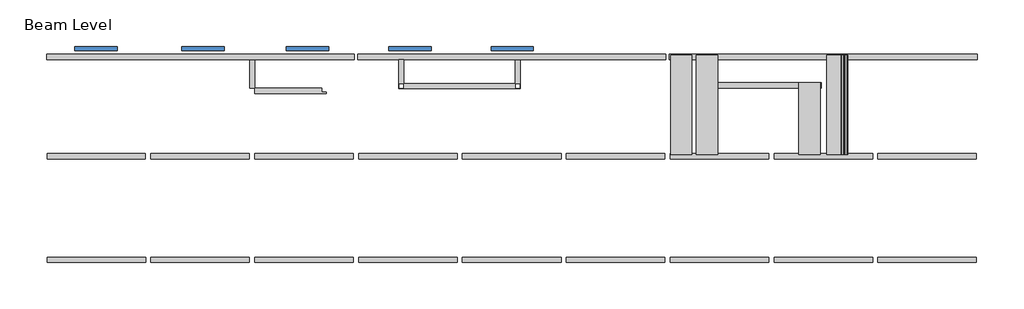
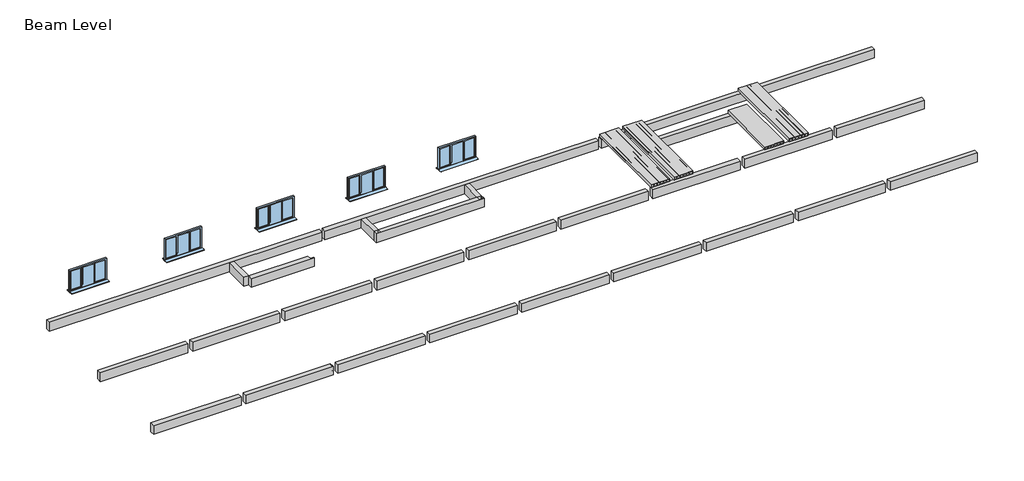
# One storey: 28 beams, 5 windows, 4 proxies.
"""IFC4 building model written with IfcOpenShell, lengths in millimetres."""

import ifcopenshell
import ifcopenshell.guid

model = None  # the IFC model being written
_history = None  # IfcOwnerHistory: only IFC2X3 demands one
_inside = {}  # id of a spatial element -> (the spatial element, [elements in it])
_under = {}  # id of a project, library or spatial element -> (it, [spatial elements below it])
_declared = {}  # id of a project -> (the project, [libraries it declares])
_typed = {}  # id of a type object -> (the type object, [elements of that type])
_made_of = {}  # id of a material, layer set ... -> (it, [elements and type objects made of it])


def new_model(schema):
    """Start an empty IFC model of exactly this schema.

    Asked for "IFC4X3", IfcOpenShell would pick the latest addendum, in which some entities
    have other attributes; the version numbers below select the first issue.
    IFC2X3 requires an IfcOwnerHistory on every rooted entity: one is made here for all.
    """
    global model, _history
    if schema == "IFC4X3":
        model = ifcopenshell.file(schema_version=(4, 3, 0, 0))
    else:
        model = ifcopenshell.file(schema=schema)
    _inside.clear()
    _under.clear()
    _declared.clear()
    _typed.clear()
    _made_of.clear()
    _history = None
    if model.schema == "IFC2X3":
        org = make("IfcOrganization", Name="unknown")
        user = make(
            "IfcPersonAndOrganization",
            ThePerson=make("IfcPerson", FamilyName="unknown"),
            TheOrganization=org,
        )
        app = make(
            "IfcApplication",
            ApplicationDeveloper=org,
            Version="unknown",
            ApplicationFullName="unknown",
            ApplicationIdentifier="unknown",
        )
        _history = make(
            "IfcOwnerHistory",
            OwningUser=user,
            OwningApplication=app,
            ChangeAction="ADDED",
            CreationDate=0,
        )
    return model


def make(cls, **values):
    """One entity of the class cls with the attributes given. An attribute that is None is left unset."""
    return model.create_entity(
        cls, **{name: value for name, value in values.items() if value is not None}
    )


def rooted(cls, **values):
    """An entity with a GlobalId (a new one), such as an element, a storey or a relation."""
    return make(cls, GlobalId=ifcopenshell.guid.new(), OwnerHistory=_history, **values)


def si_unit(unit_type, name, prefix=None):
    """IfcSIUnit, for example si_unit("LENGTHUNIT", "METRE", prefix="MILLI")."""
    return make("IfcSIUnit", UnitType=unit_type, Prefix=prefix, Name=name)


def assignment(units):
    """IfcUnitAssignment: the units of a project."""
    return None if units is None else make("IfcUnitAssignment", Units=units)


def point(xyz):
    """IfcCartesianPoint."""
    return None if xyz is None else make("IfcCartesianPoint", Coordinates=xyz)


def direction(xyz):
    """IfcDirection."""
    return None if xyz is None else make("IfcDirection", DirectionRatios=xyz)


def frame(location, z_axis=None, x_axis=None):
    """IfcAxis2Placement3D, a coordinate frame: its origin and axes. An axis left out is left unset."""
    return make(
        "IfcAxis2Placement3D",
        Location=point(location),
        Axis=direction(z_axis),
        RefDirection=direction(x_axis),
    )


def frame_2d(location, x_axis=None):
    """IfcAxis2Placement2D, a coordinate frame in the plane: its origin and x axis."""
    return make(
        "IfcAxis2Placement2D", Location=point(location), RefDirection=direction(x_axis)
    )


def origin():
    """The frame at (0, 0, 0) with its axes left unset."""
    return frame((0.0, 0.0, 0.0))


def place(relative_to, where):
    """IfcLocalPlacement: puts the frame where relative to a parent placement (None: the world)."""
    return make(
        "IfcLocalPlacement", PlacementRelTo=relative_to, RelativePlacement=where
    )


def context(
    kind, dimensions, precision=None, world=None, true_north=None, identifier=None
):
    """IfcGeometricRepresentationContext, for example the 3D "Model" context."""
    return make(
        "IfcGeometricRepresentationContext",
        ContextIdentifier=identifier,
        ContextType=kind,
        CoordinateSpaceDimension=dimensions,
        Precision=precision,
        WorldCoordinateSystem=world,
        TrueNorth=true_north,
    )


def project(units=None, contexts=None):
    """IfcProject with its units and contexts."""
    return rooted(
        "IfcProject",
        Name="project",
        RepresentationContexts=contexts,
        UnitsInContext=assignment(units),
    )


def spatial(cls, under=None, at=None, **own):
    """A site, building, storey or space (cls), placed at a placement, below another one or the project."""
    s = rooted(cls, ObjectPlacement=at, **own)
    if under is not None:
        _under.setdefault(under.id(), (under, []))[1].append(s)
    return s


def polyline(points):
    """IfcPolyline through the points."""
    return make("IfcPolyline", Points=[point(p) for p in points])


def circle_curve(where, radius):
    """IfcCircle in the frame where."""
    return make("IfcCircle", Position=where, Radius=radius)


def trimmed(basis, trim1, trim2, sense, master):
    """IfcTrimmedCurve: the piece of a basis curve between two trims."""
    return make(
        "IfcTrimmedCurve",
        BasisCurve=basis,
        Trim1=trim1,
        Trim2=trim2,
        SenseAgreement=sense,
        MasterRepresentation=master,
    )


def segment(curve, same_sense, transition):
    """IfcCompositeCurveSegment."""
    return make(
        "IfcCompositeCurveSegment",
        Transition=transition,
        SameSense=same_sense,
        ParentCurve=curve,
    )


def composite_curve(segments, self_intersect=None):
    """IfcCompositeCurve: segments joined end to end."""
    return make("IfcCompositeCurve", Segments=segments, SelfIntersect=self_intersect)


def outline(outer, holes=None, kind="AREA"):
    """IfcArbitraryClosedProfileDef: a profile drawn as a closed curve; with holes, ...WithVoids."""
    if holes is None:
        return make("IfcArbitraryClosedProfileDef", ProfileType=kind, OuterCurve=outer)
    return make(
        "IfcArbitraryProfileDefWithVoids",
        ProfileType=kind,
        OuterCurve=outer,
        InnerCurves=holes,
    )


def extrude(swept, where, along, depth):
    """IfcExtrudedAreaSolid: the profile swept, set in the frame where, extruded along a direction by depth."""
    return make(
        "IfcExtrudedAreaSolid",
        SweptArea=swept,
        Position=where,
        ExtrudedDirection=direction(along),
        Depth=depth,
    )


def faces_of(points, faces, orient=None, outer=None):
    """IfcFace entities. A face is a list of loops; a loop is a list of indices into points, from 0.

    orient and outer hold one flag for each loop. By default every Orientation is true, the
    first loop of a face is its IfcFaceOuterBound and the others are IfcFaceBound.
    """
    made = []
    for i, loops in enumerate(faces):
        bounds = []
        for j, loop in enumerate(loops):
            is_outer = j == 0 if outer is None else outer[i][j]
            bounds.append(
                make(
                    "IfcFaceOuterBound" if is_outer else "IfcFaceBound",
                    Bound=make("IfcPolyLoop", Polygon=[points[k] for k in loop]),
                    Orientation=True if orient is None else orient[i][j],
                )
            )
        made.append(make("IfcFace", Bounds=bounds))
    return made


def faceted_brep(points, faces, orient=None, outer=None, voids=None):
    """IfcFacetedBrep: a solid bounded by flat faces; with voids (closed shells), ...WithVoids."""
    shared = [point(p) for p in points]
    hull = make("IfcClosedShell", CfsFaces=faces_of(shared, faces, orient, outer))
    if voids is None:
        return make("IfcFacetedBrep", Outer=hull)
    return make(
        "IfcFacetedBrepWithVoids",
        Outer=hull,
        Voids=[
            make(cls, CfsFaces=faces_of(shared, fs, o, b)) for cls, fs, o, b in voids
        ],
    )


def shape(context_of_items, identifier, shape_type, items):
    """IfcShapeRepresentation: the items that make up one representation, for example the "Body"."""
    return make(
        "IfcShapeRepresentation",
        ContextOfItems=context_of_items,
        RepresentationIdentifier=identifier,
        RepresentationType=shape_type,
        Items=items,
    )


def source(mapping_origin, context_of_items, identifier, shape_type, items):
    """IfcRepresentationMap: a shape defined once, which mapped items show again and again."""
    return make(
        "IfcRepresentationMap",
        MappingOrigin=mapping_origin,
        MappedRepresentation=shape(context_of_items, identifier, shape_type, items),
    )


def transform(
    local_origin,
    x_axis=None,
    y_axis=None,
    z_axis=None,
    scale=None,
    scale2=None,
    scale3=None,
    uniform=True,
):
    """IfcCartesianTransformationOperator3D, or its non-uniform kind. x_axis, y_axis, z_axis: its Axis1, 2, 3."""
    if uniform:
        return make(
            "IfcCartesianTransformationOperator3D",
            Axis1=direction(x_axis),
            Axis2=direction(y_axis),
            LocalOrigin=point(local_origin),
            Scale=scale,
            Axis3=direction(z_axis),
        )
    return make(
        "IfcCartesianTransformationOperator3DnonUniform",
        Axis1=direction(x_axis),
        Axis2=direction(y_axis),
        LocalOrigin=point(local_origin),
        Scale=scale,
        Axis3=direction(z_axis),
        Scale2=scale2,
        Scale3=scale3,
    )


def mapped(mapping_source, mapping_target):
    """IfcMappedItem: shows the shape of a source again, moved by a transform."""
    return make(
        "IfcMappedItem", MappingSource=mapping_source, MappingTarget=mapping_target
    )


def made_of(thing, what):
    """Note that an element or type object is made of a material, layer set ...; save() writes the relation."""
    if what is not None:
        _made_of.setdefault(what.id(), (what, []))[1].append(thing)
    return thing


def element(
    cls,
    number,
    at=None,
    inside=None,
    cuts=None,
    type_object=None,
    material=None,
    context=None,
    identifier="Body",
    shape_type=None,
    held_by="IfcProductDefinitionShape",
    body=None,
    shapes=None,
    **own,
):
    """One element of the class cls, such as IfcWall. Its Tag is "e" and its number.

    at: its placement. inside: the storey or other place that contains it. cuts: it is an
    opening in that element (IfcRelVoidsElement). A single representation is given by context,
    identifier, shape_type and body (its items); several are given by shapes. held_by: the class
    of the entity that holds the representations. save() writes the other relations.
    """
    e = rooted(cls, Tag="e%d" % number, ObjectPlacement=at, **own)
    if body is not None:
        shapes = [shape(context, identifier, shape_type, body)]
    if shapes is not None:
        e.Representation = make(held_by, Representations=shapes)
    if inside is not None:
        _inside.setdefault(inside.id(), (inside, []))[1].append(e)
    if cuts is not None:
        rooted(
            "IfcRelVoidsElement", RelatingBuildingElement=cuts, RelatedOpeningElement=e
        )
    if type_object is not None:
        _typed.setdefault(type_object.id(), (type_object, []))[1].append(e)
    return made_of(e, material)


def aggregate(whole, parts):
    """IfcRelAggregates: a whole, such as a stair, and the parts it consists of."""
    return rooted("IfcRelAggregates", RelatingObject=whole, RelatedObjects=parts)


def save(model, path):
    """Write the relations noted so far, then the file.

    IfcRelAggregates (storeys below a building ...), IfcRelContainedInSpatialStructure (elements
    in a storey), IfcRelDefinesByType, IfcRelAssociatesMaterial and IfcRelDeclares: one each for
    every whole, place, type object, material and project.
    """
    for whole, parts in _under.values():
        aggregate(whole, parts)
    for where, things in _inside.values():
        rooted(
            "IfcRelContainedInSpatialStructure",
            RelatedElements=things,
            RelatingStructure=where,
        )
    for kind, things in _typed.values():
        rooted("IfcRelDefinesByType", RelatedObjects=things, RelatingType=kind)
    for what, things in _made_of.values():
        rooted("IfcRelAssociatesMaterial", RelatedObjects=things, RelatingMaterial=what)
    for by, libraries in _declared.values():
        rooted("IfcRelDeclares", RelatingContext=by, RelatedDefinitions=libraries)
    model.write(path)


def asb_beams_300asb153_cd404b0f(model_context):
    return source(origin(), model_context, "Body", "SweptSolid", [
        extrude(outline(composite_curve([segment(polyline([(95.0, 174.0), (95.0, 150.0), (40.5, 150.0)]), True, "CONTINUOUS"), segment(trimmed(circle_curve(frame_2d((40.5, 123.0)), 27.0), [point((40.5, 150.0))], [point((13.5, 123.0))], True, "CARTESIAN"), True, "CONTINUOUS"), segment(polyline([(13.5, 123.0), (13.5, -85.0)]), True, "CONTINUOUS"), segment(trimmed(circle_curve(frame_2d((40.5, -85.0)), 27.0), [point((13.5, -85.0))], [point((40.5, -112.0))], True, "CARTESIAN"), True, "CONTINUOUS"), segment(polyline([(40.5, -112.0), (150.0, -112.0), (150.0, -136.0), (-150.0, -136.0), (-150.0, -112.0), (-40.5, -112.0)]), True, "CONTINUOUS"), segment(trimmed(circle_curve(frame_2d((-40.5, -85.0)), 27.0), [point((-40.5, -112.0))], [point((-13.5, -85.0))], True, "CARTESIAN"), True, "CONTINUOUS"), segment(polyline([(-13.5, -85.0), (-13.5, 123.0)]), True, "CONTINUOUS"), segment(trimmed(circle_curve(frame_2d((-40.5, 123.0)), 27.0), [point((-13.5, 123.0))], [point((-40.5, 150.0))], True, "CARTESIAN"), True, "CONTINUOUS"), segment(polyline([(-40.5, 150.0), (-95.0, 150.0), (-95.0, 174.0), (95.0, 174.0)]), True, "CONTINUOUS")], self_intersect=False)), frame((-176.5, 0.0, 0.0), z_axis=(1.0, 0.0, 0.0), x_axis=(0.0, 1.0, 0.0)), (0.0, 0.0, 1.0), 36.0),
    ])


def hollow_core_b1c9e8cf(model_context):
    return source(origin(), model_context, "Body", "SweptSolid", [
        extrude(outline(polyline([(-609.6, 100.0), (609.6, 100.0), (609.6, -100.0), (-609.6, -100.0), (-609.6, 100.0)]), holes=[composite_curve([segment(trimmed(circle_curve(frame_2d((508.0, 0.0)), 60.0), [point((448.0, 0.0))], [point((568.0, 0.0))], True, "CARTESIAN"), True, "CONTINUOUS"), segment(trimmed(circle_curve(frame_2d((508.0, 0.0)), 60.0), [point((568.0, 0.0))], [point((448.0, 0.0))], True, "CARTESIAN"), True, "CONTINUOUS")], self_intersect=False), composite_curve([segment(trimmed(circle_curve(frame_2d((-508.0, 0.0)), 60.0), [point((-568.0, 0.0))], [point((-448.0, 0.0))], True, "CARTESIAN"), True, "CONTINUOUS"), segment(trimmed(circle_curve(frame_2d((-508.0, 0.0)), 60.0), [point((-448.0, 0.0))], [point((-568.0, 0.0))], True, "CARTESIAN"), True, "CONTINUOUS")], self_intersect=False), composite_curve([segment(trimmed(circle_curve(frame_2d((304.8, 0.0)), 60.0), [point((244.8, 0.0))], [point((364.8, 0.0))], True, "CARTESIAN"), True, "CONTINUOUS"), segment(trimmed(circle_curve(frame_2d((304.8, 0.0)), 60.0), [point((364.8, 0.0))], [point((244.8, 0.0))], True, "CARTESIAN"), True, "CONTINUOUS")], self_intersect=False), composite_curve([segment(trimmed(circle_curve(frame_2d((101.6, 0.0)), 60.0), [point((41.6, 0.0))], [point((161.6, 0.0))], True, "CARTESIAN"), True, "CONTINUOUS"), segment(trimmed(circle_curve(frame_2d((101.6, 0.0)), 60.0), [point((161.6, 0.0))], [point((41.6, 0.0))], True, "CARTESIAN"), True, "CONTINUOUS")], self_intersect=False), composite_curve([segment(trimmed(circle_curve(frame_2d((-101.6, 0.0)), 60.0), [point((-161.6, 0.0))], [point((-41.6, 0.0))], True, "CARTESIAN"), True, "CONTINUOUS"), segment(trimmed(circle_curve(frame_2d((-101.6, 0.0)), 60.0), [point((-41.6, 0.0))], [point((-161.6, 0.0))], True, "CARTESIAN"), True, "CONTINUOUS")], self_intersect=False), composite_curve([segment(trimmed(circle_curve(frame_2d((-304.8, 0.0)), 60.0), [point((-364.8, 0.0))], [point((-244.8, 0.0))], True, "CARTESIAN"), True, "CONTINUOUS"), segment(trimmed(circle_curve(frame_2d((-304.8, 0.0)), 60.0), [point((-244.8, 0.0))], [point((-364.8, 0.0))], True, "CARTESIAN"), True, "CONTINUOUS")], self_intersect=False)]), frame((0.0, 0.0, 0.0), z_axis=(1.0, 0.0, 0.0), x_axis=(0.0, 1.0, 0.0)), (0.0, 0.0, 1.0), 5760.0),
    ])


def hollow_core_a6975cb3(model_context):
    return source(origin(), model_context, "Body", "SweptSolid", [
        extrude(outline(polyline([(-609.6, 100.0), (609.6, 100.0), (609.6, -100.0), (-609.6, -100.0), (-609.6, 100.0)]), holes=[composite_curve([segment(trimmed(circle_curve(frame_2d((508.0, 0.0)), 60.0), [point((448.0, 0.0))], [point((568.0, 0.0))], True, "CARTESIAN"), True, "CONTINUOUS"), segment(trimmed(circle_curve(frame_2d((508.0, 0.0)), 60.0), [point((568.0, 0.0))], [point((448.0, 0.0))], True, "CARTESIAN"), True, "CONTINUOUS")], self_intersect=False), composite_curve([segment(trimmed(circle_curve(frame_2d((-508.0, 0.0)), 60.0), [point((-568.0, 0.0))], [point((-448.0, 0.0))], True, "CARTESIAN"), True, "CONTINUOUS"), segment(trimmed(circle_curve(frame_2d((-508.0, 0.0)), 60.0), [point((-448.0, 0.0))], [point((-568.0, 0.0))], True, "CARTESIAN"), True, "CONTINUOUS")], self_intersect=False), composite_curve([segment(trimmed(circle_curve(frame_2d((304.8, 0.0)), 60.0), [point((244.8, 0.0))], [point((364.8, 0.0))], True, "CARTESIAN"), True, "CONTINUOUS"), segment(trimmed(circle_curve(frame_2d((304.8, 0.0)), 60.0), [point((364.8, 0.0))], [point((244.8, 0.0))], True, "CARTESIAN"), True, "CONTINUOUS")], self_intersect=False), composite_curve([segment(trimmed(circle_curve(frame_2d((101.6, 0.0)), 60.0), [point((41.6, 0.0))], [point((161.6, 0.0))], True, "CARTESIAN"), True, "CONTINUOUS"), segment(trimmed(circle_curve(frame_2d((101.6, 0.0)), 60.0), [point((161.6, 0.0))], [point((41.6, 0.0))], True, "CARTESIAN"), True, "CONTINUOUS")], self_intersect=False), composite_curve([segment(trimmed(circle_curve(frame_2d((-101.6, 0.0)), 60.0), [point((-161.6, 0.0))], [point((-41.6, 0.0))], True, "CARTESIAN"), True, "CONTINUOUS"), segment(trimmed(circle_curve(frame_2d((-101.6, 0.0)), 60.0), [point((-41.6, 0.0))], [point((-161.6, 0.0))], True, "CARTESIAN"), True, "CONTINUOUS")], self_intersect=False), composite_curve([segment(trimmed(circle_curve(frame_2d((-304.8, 0.0)), 60.0), [point((-364.8, 0.0))], [point((-244.8, 0.0))], True, "CARTESIAN"), True, "CONTINUOUS"), segment(trimmed(circle_curve(frame_2d((-304.8, 0.0)), 60.0), [point((-244.8, 0.0))], [point((-364.8, 0.0))], True, "CARTESIAN"), True, "CONTINUOUS")], self_intersect=False)]), frame((0.0, 0.0, 0.0), z_axis=(1.0, 0.0, 0.0), x_axis=(0.0, 1.0, 0.0)), (0.0, 0.0, 1.0), 4157.5),
    ])


def windows_commercial_ff_rear_windows_2400long_x_1500high_d88e899e(model_context):
    return source(origin(), model_context, "Body", "SolidModel", [
        extrude(outline(polyline([(-1860.0, -231.5434322), (-1860.0, -138.5434322), (-1860.0, 8.4565678), (590.0, 8.4565678), (590.0, -138.5434322), (590.0, -231.5434322), (-1860.0, -231.5434322)])), frame((0.0, 0.0, 636.5715519), z_axis=(0.0, 0.0, 1.0), x_axis=(1.0, 0.0, 0.0)), (0.0, 0.0, 1.0), 26.4284481),
        extrude(outline(polyline([(495.0, 87.4565678), (-190.0, 87.4565678), (-190.0, 111.4565678), (495.0, 111.4565678), (495.0, 87.4565678)])), frame((0.0, 0.0, 693.0), z_axis=(0.0, 0.0, 1.0), x_axis=(1.0, 0.0, 0.0)), (0.0, 0.0, 1.0), 1337.0),
        extrude(outline(polyline([(-1020.0, 47.4565678), (-250.0, 47.4565678), (-250.0, 23.4565678), (-1020.0, 23.4565678), (-1020.0, 47.4565678)])), frame((0.0, 0.0, 663.0), z_axis=(0.0, 0.0, 1.0), x_axis=(1.0, 0.0, 0.0)), (0.0, 0.0, 1.0), 1397.0),
        extrude(outline(polyline([(-1080.0, 87.4565678), (-1765.0, 87.4565678), (-1765.0, 111.4565678), (-1080.0, 111.4565678), (-1080.0, 87.4565678)])), frame((0.0, 0.0, 693.0), z_axis=(0.0, 0.0, 1.0), x_axis=(1.0, 0.0, 0.0)), (0.0, 0.0, 1.0), 1337.0),
        faceted_brep([(-1835.0, 5.4565678, 663.0), (-1775.0, 5.4565678, 663.0), (-1775.0, 5.4565678, 2040.0), (-1068.0, 5.4565678, 2040.0), (-1068.0, 5.4565678, 863.0), (-1010.0, 5.4565678, 863.0), (-1010.0, 5.4565678, 2040.0), (-260.0, 5.4565678, 2040.0), (-260.0, 5.4565678, 663.0), (-202.0, 5.4565678, 663.0), (-202.0, 5.4565678, 2040.0), (505.0, 5.4565678, 2040.0), (505.0, 5.4565678, 663.0), (565.0, 5.4565678, 663.0), (565.0, 5.4565678, 2100.0), (-1835.0, 5.4565678, 2100.0), (-1835.0, 123.4565678, 2100.0), (-1835.0, 123.4565678, 663.0), (-1835.0, 73.4565678, 663.0), (-1835.0, 8.4565678, 663.0), (-1795.0, 123.4565678, 663.0), (565.0, 123.4565678, 2100.0), (565.0, 123.4565678, 663.0), (525.0, 123.4565678, 663.0), (525.0, 123.4565678, 2060.0), (-220.0, 123.4565678, 2060.0), (-220.0, 123.4565678, 663.0), (-260.0, 123.4565678, 663.0), (-260.0, 123.4565678, 2060.0), (-1010.0, 123.4565678, 2060.0), (-1010.0, 123.4565678, 863.0), (-1050.0, 123.4565678, 863.0), (-1050.0, 123.4565678, 2060.0), (-1795.0, 123.4565678, 2060.0), (-1795.0, 23.4565678, 2060.0), (-1795.0, 23.4565678, 663.0), (-1795.0, 73.4565678, 663.0), (-1050.0, 23.4565678, 2060.0), (-1050.0, 23.4565678, 863.0), (-1068.0, 23.4565678, 863.0), (-1068.0, 23.4565678, 2040.0), (-1775.0, 23.4565678, 2040.0), (-1775.0, 23.4565678, 663.0), (525.0, 23.4565678, 2060.0), (525.0, 23.4565678, 663.0), (505.0, 23.4565678, 663.0), (505.0, 23.4565678, 2040.0), (-202.0, 23.4565678, 2040.0), (-202.0, 23.4565678, 663.0), (-220.0, 23.4565678, 663.0), (-220.0, 23.4565678, 2060.0), (-1010.0, 23.4565678, 863.0), (-1020.0, 23.4565678, 863.0), (-1020.0, 23.4565678, 2060.0), (-250.0, 23.4565678, 2060.0), (-250.0, 23.4565678, 663.0), (-260.0, 23.4565678, 663.0), (-260.0, 23.4565678, 2040.0), (-1010.0, 23.4565678, 2040.0), (-1775.0, 8.4565678, 663.0), (-1010.0, 47.4565678, 2060.0), (-260.0, 47.4565678, 2060.0), (-250.0, 47.4565678, 2060.0), (-1020.0, 47.4565678, 2060.0), (565.0, 8.4565678, 663.0), (565.0, 73.4565678, 663.0), (525.0, 73.4565678, 663.0), (505.0, 8.4565678, 663.0), (-1010.0, 47.4565678, 863.0), (-1020.0, 47.4565678, 863.0), (-250.0, 47.4565678, 663.0), (-260.0, 47.4565678, 663.0), (-260.0, 73.4565678, 663.0), (-220.0, 73.4565678, 663.0), (-202.0, 8.4565678, 663.0), (-260.0, 8.4565678, 663.0), (590.0, 248.4565678, 600.0), (590.0, 8.4565678, 600.0), (-1860.0, 8.4565678, 600.0), (-1860.0, 248.4565678, 600.0), (590.0, 248.4565678, 637.0666405), (-1860.0, 248.4565678, 637.0666405), (590.0, 73.4565678, 649.0962075), (-1860.0, 73.4565678, 649.0962075), (590.0, 8.4565678, 663.0), (590.0, 73.4565678, 663.0), (-1860.0, 73.4565678, 663.0), (-1860.0, 8.4565678, 663.0)], [[[0, 1, 2, 3, 4, 5, 6, 7, 8, 9, 10, 11, 12, 13, 14, 15]], [[0, 15, 16, 17, 18, 19]], [[20, 17, 16, 21, 22, 23, 24, 25, 26, 27, 28, 29, 30, 31, 32, 33]], [[20, 33, 34, 35, 36]], [[35, 34, 37, 38, 39, 40, 41, 42]], [[43, 44, 45, 46, 47, 48, 49, 50]], [[51, 52, 53, 54, 55, 56, 57, 58]], [[2, 1, 59, 42, 41]], [[15, 14, 21, 16]], [[34, 33, 32, 37]], [[24, 43, 50, 25]], [[60, 29, 28, 61, 62, 54, 53, 63]], [[2, 41, 40, 3]], [[46, 11, 10, 47]], [[6, 58, 57, 7]], [[14, 13, 64, 65, 22, 21]], [[24, 23, 66, 44, 43]], [[12, 11, 46, 45, 67]], [[5, 51, 58, 6]], [[39, 4, 3, 40]], [[31, 38, 37, 32]], [[68, 30, 29, 60]], [[69, 68, 60, 63]], [[52, 69, 63, 53]], [[62, 70, 55, 54]], [[70, 62, 61, 71]], [[71, 61, 28, 27, 72]], [[26, 25, 50, 49, 73]], [[10, 9, 74, 48, 47]], [[8, 7, 57, 56, 75]], [[76, 77, 78, 79]], [[80, 76, 79, 81]], [[82, 80, 81, 83]], [[84, 85, 65, 64]], [[86, 87, 19, 18]], [[72, 36, 35, 42, 59, 75, 56, 55, 70, 71]], [[66, 73, 49, 48, 74, 67, 45, 44]], [[17, 20, 36, 18]], [[1, 0, 19, 59]], [[23, 22, 65, 66]], [[13, 12, 67, 64]], [[51, 5, 4, 39, 38, 31, 30, 68, 69, 52]], [[27, 26, 73, 72]], [[9, 8, 75, 74]], [[84, 77, 76, 80, 82, 85]], [[87, 86, 83, 81, 79, 78]], [[85, 82, 83, 86, 18, 36, 72, 73, 66, 65]], [[77, 84, 64, 67, 74, 75, 59, 19, 87, 78]]]),
        faceted_brep([(-1050.0, 23.4565678, 2060.0), (-1050.0, 93.4565678, 2060.0), (-1795.0, 93.4565678, 2060.0), (-1795.0, 23.4565678, 2060.0), (-1090.0, 37.9494677, 2020.0), (-1079.8519623, 23.4565678, 2030.1480377), (-1765.1480377, 23.4565678, 2030.1480377), (-1755.0, 37.9494677, 2020.0), (-1090.0, 87.4565678, 2020.0), (-1755.0, 87.4565678, 2020.0), (-1080.0, 111.4565678, 2030.0), (-1080.0, 87.4565678, 2030.0), (-1765.0, 87.4565678, 2030.0), (-1765.0, 111.4565678, 2030.0), (-1090.0, 129.2300705, 2020.0), (-1090.0, 111.4565678, 2020.0), (-1755.0, 111.4565678, 2020.0), (-1755.0, 129.2300705, 2020.0), (-1071.1854344, 135.0035732, 2038.8145656), (-1773.8145656, 135.0035732, 2038.8145656), (-1795.0, 93.4565678, 663.0), (-1795.0, 23.4565678, 663.0), (-1765.1480377, 23.4565678, 692.8519623), (-1755.0, 37.9494677, 703.0), (-1755.0, 87.4565678, 703.0), (-1765.0, 87.4565678, 693.0), (-1765.0, 111.4565678, 693.0), (-1755.0, 111.4565678, 703.0), (-1755.0, 129.2300705, 703.0), (-1773.8145656, 135.0035732, 684.1854344), (-1050.0, 93.4565678, 663.0), (-1050.0, 23.4565678, 663.0), (-1079.8519623, 23.4565678, 692.8519623), (-1090.0, 37.9494677, 703.0), (-1090.0, 87.4565678, 703.0), (-1080.0, 87.4565678, 693.0), (-1080.0, 111.4565678, 693.0), (-1090.0, 111.4565678, 703.0), (-1090.0, 129.2300705, 703.0), (-1071.1854344, 135.0035732, 684.1854344), (-1040.0, 135.0035732, 653.0), (-1805.0, 135.0035732, 653.0), (-1805.0, 135.0035732, 2070.0), (-1040.0, 135.0035732, 2070.0), (-1040.0, 93.4565678, 2070.0), (-1805.0, 93.4565678, 2070.0), (-1805.0, 93.4565678, 653.0), (-1040.0, 93.4565678, 653.0)], [[[0, 1, 2, 3]], [[4, 5, 6, 7]], [[8, 4, 7, 9]], [[10, 11, 12, 13]], [[14, 15, 16, 17]], [[18, 14, 17, 19]], [[3, 2, 20, 21]], [[7, 6, 22, 23]], [[9, 7, 23, 24]], [[13, 12, 25, 26]], [[17, 16, 27, 28]], [[19, 17, 28, 29]], [[21, 20, 30, 31]], [[0, 3, 21, 31], [32, 22, 6, 5]], [[23, 22, 32, 33]], [[24, 23, 33, 34]], [[35, 25, 12, 11], [8, 9, 24, 34]], [[26, 25, 35, 36]], [[10, 13, 26, 36], [37, 27, 16, 15]], [[28, 27, 37, 38]], [[29, 28, 38, 39]], [[40, 41, 42, 43], [18, 19, 29, 39]], [[30, 1, 0, 31]], [[33, 32, 5, 4]], [[34, 33, 4, 8]], [[36, 35, 11, 10]], [[38, 37, 15, 14]], [[39, 38, 14, 18]], [[44, 43, 42, 45]], [[45, 42, 41, 46]], [[46, 41, 40, 47]], [[47, 40, 43, 44]], [[45, 46, 47, 44], [1, 30, 20, 2]]]),
        faceted_brep([(-230.0, 87.4565678, 2070.0), (-230.0, 129.2300705, 2070.0), (-230.0, 129.2300705, 653.0), (-230.0, 87.4565678, 653.0), (-220.0, 23.4565678, 2060.0), (-220.0, 87.4565678, 2060.0), (-220.0, 87.4565678, 663.0), (-220.0, 23.4565678, 663.0), (-180.0, 37.9494677, 2020.0), (-190.1480377, 23.4565678, 2030.1480377), (-190.1480377, 23.4565678, 692.8519623), (-180.0, 37.9494677, 703.0), (-180.0, 87.4565678, 2020.0), (-180.0, 87.4565678, 703.0), (-190.0, 111.4565678, 2030.0), (-190.0, 87.4565678, 2030.0), (-190.0, 87.4565678, 693.0), (-190.0, 111.4565678, 693.0), (-180.0, 129.2300705, 2020.0), (-180.0, 111.4565678, 2020.0), (-180.0, 111.4565678, 703.0), (-180.0, 129.2300705, 703.0), (-197.4457548, 135.0035732, 2037.4457548), (-197.4457548, 135.0035732, 685.5542452), (-219.2153903, 135.0035732, 2059.2153903), (-219.2153903, 135.0035732, 663.7846097), (535.0, 129.2300705, 653.0), (535.0, 87.4565678, 653.0), (525.0, 87.4565678, 663.0), (525.0, 23.4565678, 663.0), (495.1480377, 23.4565678, 692.8519623), (485.0, 37.9494677, 703.0), (485.0, 87.4565678, 703.0), (495.0, 87.4565678, 693.0), (495.0, 111.4565678, 693.0), (485.0, 111.4565678, 703.0), (485.0, 129.2300705, 703.0), (502.4457548, 135.0035732, 685.5542452), (524.2153903, 135.0035732, 663.7846097), (535.0, 129.2300705, 2070.0), (535.0, 87.4565678, 2070.0), (525.0, 87.4565678, 2060.0), (525.0, 23.4565678, 2060.0), (495.1480377, 23.4565678, 2030.1480377), (485.0, 37.9494677, 2020.0), (485.0, 87.4565678, 2020.0), (495.0, 87.4565678, 2030.0), (495.0, 111.4565678, 2030.0), (485.0, 111.4565678, 2020.0), (485.0, 129.2300705, 2020.0), (502.4457548, 135.0035732, 2037.4457548), (524.2153903, 135.0035732, 2059.2153903)], [[[0, 1, 2, 3]], [[4, 5, 6, 7]], [[8, 9, 10, 11]], [[12, 8, 11, 13]], [[14, 15, 16, 17]], [[18, 19, 20, 21]], [[22, 18, 21, 23]], [[1, 24, 25, 2]], [[3, 2, 26, 27]], [[7, 6, 28, 29]], [[11, 10, 30, 31]], [[13, 11, 31, 32]], [[17, 16, 33, 34]], [[21, 20, 35, 36]], [[23, 21, 36, 37]], [[2, 25, 38, 26]], [[27, 26, 39, 40]], [[29, 28, 41, 42]], [[31, 30, 43, 44]], [[32, 31, 44, 45]], [[34, 33, 46, 47]], [[36, 35, 48, 49]], [[37, 36, 49, 50]], [[26, 38, 51, 39]], [[40, 39, 1, 0]], [[42, 41, 5, 4]], [[7, 29, 42, 4], [9, 43, 30, 10]], [[44, 43, 9, 8]], [[45, 44, 8, 12]], [[15, 46, 33, 16], [13, 32, 45, 12]], [[47, 46, 15, 14]], [[17, 34, 47, 14], [19, 48, 35, 20]], [[49, 48, 19, 18]], [[50, 49, 18, 22]], [[24, 51, 38, 25], [23, 37, 50, 22]], [[39, 51, 24, 1]], [[3, 27, 40, 0], [5, 41, 28, 6]]]),
    ])


model = new_model("IFC4")

# Units and contexts
model_context = context("Model", 3, world=origin())
ifc_project = project(units=[si_unit("LENGTHUNIT", "METRE", prefix="MILLI")], contexts=[model_context])

# Site, building, storey
site = spatial("IfcSite", under=ifc_project)
building = spatial("IfcBuilding", under=site)
storey = spatial("IfcBuildingStorey", under=building, Name="Beam Level", Elevation=3700.0)

# Beams
placement = place(None, origin())
asb_beams_300asb153_shape = asb_beams_300asb153_cd404b0f(model_context)
element("IfcBeam", 1, ObjectType="ASB-Beams : 300ASB153", at=placement, inside=storey, context=model_context, shape_type="MappedRepresentation", body=[
    mapped(asb_beams_300asb153_shape, transform((4837.4196543, -5058.7619082, 3526.0), x_axis=(1.0, 0.0, 0.0), y_axis=(0.0, 1.0, 0.0), z_axis=(0.0, 0.0, 1.0))),
])
element("IfcBeam", 2, ObjectType="Concrete - Rectangular Beam : 300 x 600mm", at=placement, inside=storey, context=model_context, shape_type="SweptSolid", body=[
    extrude(outline(polyline([(-1300.8053457, 1091.2380918), (-1300.8053457, 791.2380918), (-6985.5053457, 791.2380918), (-6985.5053457, 1091.2380918), (-1300.8053457, 1091.2380918)])), frame((0.0, 0.0, 3100.0), z_axis=(0.0, 0.0, 1.0), x_axis=(1.0, 0.0, 0.0)), (0.0, 0.0, 1.0), 600.0),
])
element("IfcBeam", 3, ObjectType="Concrete - Rectangular Beam : 300 x 600mm", at=placement, inside=storey, context=model_context, shape_type="SweptSolid", body=[
    extrude(outline(polyline([(-985.6053457, 791.2380918), (-985.6053457, 1091.2380918), (4710.4446543, 1091.2380918), (4710.4446543, 791.2380918), (-985.6053457, 791.2380918)])), frame((0.0, 0.0, 3100.0), z_axis=(0.0, 0.0, 1.0), x_axis=(1.0, 0.0, 0.0)), (0.0, 0.0, 1.0), 600.0),
])
element("IfcBeam", 4, ObjectType="Concrete - Rectangular Beam : 300 x 600mm", at=placement, inside=storey, context=model_context, shape_type="SweptSolid", body=[
    extrude(outline(polyline([(10706.1946543, 1091.2380918), (10706.1946543, 791.2380918), (5010.4446543, 791.2380918), (5010.4446543, 1091.2380918), (10706.1946543, 1091.2380918)])), frame((0.0, 0.0, 3100.0), z_axis=(0.0, 0.0, 1.0), x_axis=(1.0, 0.0, 0.0)), (0.0, 0.0, 1.0), 600.0),
])
element("IfcBeam", 5, ObjectType="Concrete - Rectangular Beam : 300 x 600mm", at=placement, inside=storey, context=model_context, shape_type="SweptSolid", body=[
    extrude(outline(polyline([(-6985.3053457, -5208.7619082), (-6985.3053457, -4908.7619082), (-1289.5553457, -4908.7619082), (-1289.5553457, -5208.7619082), (-6985.3053457, -5208.7619082)])), frame((0.0, 0.0, 3100.0), z_axis=(0.0, 0.0, 1.0), x_axis=(1.0, 0.0, 0.0)), (0.0, 0.0, 1.0), 600.0),
])
element("IfcBeam", 6, ObjectType="Concrete - Rectangular Beam : 300 x 600mm", at=placement, inside=storey, context=model_context, shape_type="SweptSolid", body=[
    extrude(outline(polyline([(-985.6053457, -5208.7619082), (-985.6053457, -4908.7619082), (4710.4446543, -4908.7619082), (4710.4446543, -5208.7619082), (-985.6053457, -5208.7619082)])), frame((0.0, 0.0, 3100.0), z_axis=(0.0, 0.0, 1.0), x_axis=(1.0, 0.0, 0.0)), (0.0, 0.0, 1.0), 600.0),
])
element("IfcBeam", 7, ObjectType="Concrete - Rectangular Beam : 300 x 600mm", at=placement, inside=storey, context=model_context, shape_type="SweptSolid", body=[
    extrude(outline(polyline([(10706.1946543, -4908.7619082), (10706.1946543, -5208.7619082), (5010.4446543, -5208.7619082), (5010.4446543, -4908.7619082), (10706.1946543, -4908.7619082)])), frame((0.0, 0.0, 3100.0), z_axis=(0.0, 0.0, 1.0), x_axis=(1.0, 0.0, 0.0)), (0.0, 0.0, 1.0), 600.0),
])
element("IfcBeam", 8, ObjectType="Concrete - Rectangular Beam : 300 x 600mm", at=placement, inside=storey, context=model_context, shape_type="SweptSolid", body=[
    extrude(outline(polyline([(16699.1946543, 1091.2380918), (16699.1946543, 791.2380918), (11014.4946543, 791.2380918), (11014.4946543, 1091.2380918), (16699.1946543, 1091.2380918)])), frame((0.0, 0.0, 3100.0), z_axis=(0.0, 0.0, 1.0), x_axis=(1.0, 0.0, 0.0)), (0.0, 0.0, 1.0), 600.0),
])
element("IfcBeam", 9, ObjectType="Concrete - Rectangular Beam : 300 x 600mm", at=placement, inside=storey, context=model_context, shape_type="SweptSolid", body=[
    extrude(outline(polyline([(17014.3946543, 791.2380918), (17014.3946543, 1091.2380918), (22710.4446543, 1091.2380918), (22710.4446543, 791.2380918), (17014.3946543, 791.2380918)])), frame((0.0, 0.0, 3100.0), z_axis=(0.0, 0.0, 1.0), x_axis=(1.0, 0.0, 0.0)), (0.0, 0.0, 1.0), 600.0),
])
element("IfcBeam", 10, ObjectType="Concrete - Rectangular Beam : 300 x 600mm", at=placement, inside=storey, context=model_context, shape_type="SweptSolid", body=[
    extrude(outline(polyline([(28706.1946543, 1091.2380918), (28706.1946543, 791.2380918), (23010.4446543, 791.2380918), (23010.4446543, 1091.2380918), (28706.1946543, 1091.2380918)])), frame((0.0, 0.0, 3100.0), z_axis=(0.0, 0.0, 1.0), x_axis=(1.0, 0.0, 0.0)), (0.0, 0.0, 1.0), 600.0),
])
element("IfcBeam", 11, ObjectType="Concrete - Rectangular Beam : 300 x 600mm", at=placement, inside=storey, context=model_context, shape_type="SweptSolid", body=[
    extrude(outline(polyline([(11014.6946543, -5208.7619082), (11014.6946543, -4908.7619082), (16710.4446543, -4908.7619082), (16710.4446543, -5208.7619082), (11014.6946543, -5208.7619082)])), frame((0.0, 0.0, 3100.0), z_axis=(0.0, 0.0, 1.0), x_axis=(1.0, 0.0, 0.0)), (0.0, 0.0, 1.0), 600.0),
])
element("IfcBeam", 12, ObjectType="Concrete - Rectangular Beam : 300 x 600mm", at=placement, inside=storey, context=model_context, shape_type="SweptSolid", body=[
    extrude(outline(polyline([(17014.3946543, -5208.7619082), (17014.3946543, -4908.7619082), (22710.4446543, -4908.7619082), (22710.4446543, -5208.7619082), (17014.3946543, -5208.7619082)])), frame((0.0, 0.0, 3100.0), z_axis=(0.0, 0.0, 1.0), x_axis=(1.0, 0.0, 0.0)), (0.0, 0.0, 1.0), 600.0),
])
element("IfcBeam", 13, ObjectType="Concrete - Rectangular Beam : 300 x 600mm", at=placement, inside=storey, context=model_context, shape_type="SweptSolid", body=[
    extrude(outline(polyline([(28706.1946543, -4908.7619082), (28706.1946543, -5208.7619082), (23010.4446543, -5208.7619082), (23010.4446543, -4908.7619082), (28706.1946543, -4908.7619082)])), frame((0.0, 0.0, 3100.0), z_axis=(0.0, 0.0, 1.0), x_axis=(1.0, 0.0, 0.0)), (0.0, 0.0, 1.0), 600.0),
])
element("IfcBeam", 14, ObjectType="Concrete - Rectangular Beam : 300 x 600mm", at=placement, inside=storey, context=model_context, shape_type="SweptSolid", body=[
    extrude(outline(polyline([(34699.1946543, 1091.2380918), (34699.1946543, 791.2380918), (29014.4946543, 791.2380918), (29014.4946543, 1091.2380918), (34699.1946543, 1091.2380918)])), frame((0.0, 0.0, 3100.0), z_axis=(0.0, 0.0, 1.0), x_axis=(1.0, 0.0, 0.0)), (0.0, 0.0, 1.0), 600.0),
])
element("IfcBeam", 15, ObjectType="Concrete - Rectangular Beam : 300 x 600mm", at=placement, inside=storey, context=model_context, shape_type="SweptSolid", body=[
    extrude(outline(polyline([(35014.3946543, 791.2380918), (35014.3946543, 1091.2380918), (40710.4446543, 1091.2380918), (40710.4446543, 791.2380918), (35014.3946543, 791.2380918)])), frame((0.0, 0.0, 3100.0), z_axis=(0.0, 0.0, 1.0), x_axis=(1.0, 0.0, 0.0)), (0.0, 0.0, 1.0), 600.0),
])
element("IfcBeam", 16, ObjectType="Concrete - Rectangular Beam : 300 x 600mm", at=placement, inside=storey, context=model_context, shape_type="SweptSolid", body=[
    extrude(outline(polyline([(46706.1946543, 1091.2380918), (46706.1946543, 791.2380918), (41010.4446543, 791.2380918), (41010.4446543, 1091.2380918), (46706.1946543, 1091.2380918)])), frame((0.0, 0.0, 3100.0), z_axis=(0.0, 0.0, 1.0), x_axis=(1.0, 0.0, 0.0)), (0.0, 0.0, 1.0), 600.0),
])
element("IfcBeam", 17, ObjectType="Concrete - Rectangular Beam : 300 x 600mm", at=placement, inside=storey, context=model_context, shape_type="SweptSolid", body=[
    extrude(outline(polyline([(29014.6946543, -5208.7619082), (29014.6946543, -4908.7619082), (34710.4446543, -4908.7619082), (34710.4446543, -5208.7619082), (29014.6946543, -5208.7619082)])), frame((0.0, 0.0, 3100.0), z_axis=(0.0, 0.0, 1.0), x_axis=(1.0, 0.0, 0.0)), (0.0, 0.0, 1.0), 600.0),
])
element("IfcBeam", 18, ObjectType="Concrete - Rectangular Beam : 300 x 600mm", at=placement, inside=storey, context=model_context, shape_type="SweptSolid", body=[
    extrude(outline(polyline([(35014.3946543, -5208.7619082), (35014.3946543, -4908.7619082), (40710.4446543, -4908.7619082), (40710.4446543, -5208.7619082), (35014.3946543, -5208.7619082)])), frame((0.0, 0.0, 3100.0), z_axis=(0.0, 0.0, 1.0), x_axis=(1.0, 0.0, 0.0)), (0.0, 0.0, 1.0), 600.0),
])
element("IfcBeam", 19, ObjectType="Concrete - Rectangular Beam : 300 x 600mm", at=placement, inside=storey, context=model_context, shape_type="SweptSolid", body=[
    extrude(outline(polyline([(46705.4946543, -4908.7619082), (46705.4946543, -5208.7619082), (41010.4446543, -5208.7619082), (41010.4446543, -4908.7619082), (46705.4946543, -4908.7619082)])), frame((0.0, 0.0, 3100.0), z_axis=(0.0, 0.0, 1.0), x_axis=(1.0, 0.0, 0.0)), (0.0, 0.0, 1.0), 600.0),
])
element("IfcBeam", 20, ObjectType="Concrete - Rectangular Beam : 300 x 600mm", at=placement, inside=storey, context=model_context, shape_type="Brep", body=[
    faceted_brep([(10765.2696543, 6833.7380918, 3700.0), (10765.2696543, 6533.7380918, 3700.0), (10765.2696543, 6533.7380918, 3100.0), (10765.2696543, 6833.7380918, 3100.0), (-7013.1303457, 6833.7380918, 3700.0), (-7013.1303457, 6833.7380918, 3100.0), (-7013.1303457, 6533.7380918, 3100.0), (-7013.1303457, 6533.7380918, 3700.0), (4722.9446543, 6533.7380918, 3700.0), (5022.9446543, 6533.7380918, 3700.0), (4722.9446543, 6533.7380918, 3100.0), (5022.9446543, 6533.7380918, 3100.0)], [[[0, 1, 2, 3]], [[4, 5, 6, 7]], [[1, 0, 4, 7, 8, 9]], [[2, 1, 9, 8, 7, 6, 10, 11]], [[3, 2, 11, 10, 6, 5]], [[0, 3, 5, 4]]]),
])
element("IfcBeam", 21, ObjectType="Concrete - Rectangular Beam : 300 x 600mm", at=placement, inside=storey, context=model_context, shape_type="Brep", body=[
    faceted_brep([(28765.6446543, 6833.7380918, 3700.0), (28765.6446543, 6533.7380918, 3700.0), (28765.6446543, 6533.7380918, 3100.0), (28765.6446543, 6833.7380918, 3100.0), (10960.2446543, 6833.7380918, 3700.0), (10960.2446543, 6833.7380918, 3100.0), (10960.2446543, 6533.7380918, 3100.0), (10960.2446543, 6533.7380918, 3700.0), (13322.5475614, 6533.7380918, 3700.0), (13622.5475614, 6533.7380918, 3700.0), (20056.9831159, 6533.7380918, 3700.0), (20356.9831159, 6533.7380918, 3700.0), (13322.5475614, 6533.7380918, 3100.0), (13622.5475614, 6533.7380918, 3100.0), (20056.9831159, 6533.7380918, 3100.0), (20356.9831159, 6533.7380918, 3100.0)], [[[0, 1, 2, 3]], [[4, 5, 6, 7]], [[1, 0, 4, 7, 8, 9, 10, 11]], [[2, 1, 11, 10, 9, 8, 7, 6, 12, 13, 14, 15]], [[3, 2, 15, 14, 13, 12, 6, 5]], [[0, 3, 5, 4]]]),
])
element("IfcBeam", 22, ObjectType="Concrete - Rectangular Beam : 300 x 600mm", at=placement, inside=storey, context=model_context, shape_type="SweptSolid", body=[
    extrude(outline(polyline([(9144.5066977, 4575.3001351), (5022.9446543, 4575.3001351), (5022.9446543, 4875.3001351), (8894.5066977, 4875.3001351), (8894.5066977, 4635.3001351), (9144.5066977, 4635.3001351), (9144.5066977, 4575.3001351)])), frame((0.0, 0.0, 3100.0), z_axis=(0.0, 0.0, 1.0), x_axis=(1.0, 0.0, 0.0)), (0.0, 0.0, 1.0), 600.0),
])
element("IfcBeam", 23, ObjectType="Concrete - Rectangular Beam : 300 x 600mm", at=placement, inside=storey, context=model_context, shape_type="SweptSolid", body=[
    extrude(outline(polyline([(13322.5475614, 4846.2380918), (13322.5475614, 5146.2380918), (13327.9446543, 5146.2380918), (13327.9446543, 4850.3001351), (13627.9446543, 4850.3001351), (13627.9446543, 5146.2380918), (20050.4446543, 5146.2380918), (20050.4446543, 4850.3001351), (20350.4446543, 4850.3001351), (20350.4446543, 5146.2380918), (20356.9831159, 5146.2380918), (20356.9831159, 4846.2380918), (13322.5475614, 4846.2380918)])), frame((0.0, 0.0, 3100.0), z_axis=(0.0, 0.0, 1.0), x_axis=(1.0, 0.0, 0.0)), (0.0, 0.0, 1.0), 600.0),
])
element("IfcBeam", 24, ObjectType="Concrete - Rectangular Beam : 300 x 600mm", at=placement, inside=storey, context=model_context, shape_type="SweptSolid", body=[
    extrude(outline(polyline([(13322.5475614, 6533.7380918), (13622.5475614, 6533.7380918), (13622.5475614, 5150.3001351), (13327.9446543, 5150.3001351), (13327.9446543, 5146.2380918), (13322.5475614, 5146.2380918), (13322.5475614, 6533.7380918)])), frame((0.0, 0.0, 3100.0), z_axis=(0.0, 0.0, 1.0), x_axis=(1.0, 0.0, 0.0)), (0.0, 0.0, 1.0), 600.0),
])
element("IfcBeam", 25, ObjectType="Concrete - Rectangular Beam : 300 x 600mm", at=placement, inside=storey, context=model_context, shape_type="SweptSolid", body=[
    extrude(outline(polyline([(20056.9831159, 6533.7380918), (20356.9831159, 6533.7380918), (20356.9831159, 5146.2380918), (20350.4446543, 5146.2380918), (20350.4446543, 5150.3001351), (20056.9831159, 5150.3001351), (20056.9831159, 6533.7380918)])), frame((0.0, 0.0, 3100.0), z_axis=(0.0, 0.0, 1.0), x_axis=(1.0, 0.0, 0.0)), (0.0, 0.0, 1.0), 600.0),
])
element("IfcBeam", 26, ObjectType="Concrete - Rectangular Beam : 300 x 600mm", at=placement, inside=storey, context=model_context, shape_type="SweptSolid", body=[
    extrude(outline(polyline([(5022.9446543, 6533.7380918), (5022.9446543, 4875.3001351), (4722.9446543, 4875.3001351), (4722.9446543, 6533.7380918), (5022.9446543, 6533.7380918)])), frame((0.0, 0.0, 3100.0), z_axis=(0.0, 0.0, 1.0), x_axis=(1.0, 0.0, 0.0)), (0.0, 0.0, 1.0), 600.0),
])
element("IfcBeam", 27, ObjectType="Concrete - Rectangular Beam : 300 x 600mm", at=placement, inside=storey, context=model_context, shape_type="SweptSolid", body=[
    extrude(outline(polyline([(46765.6446543, 6833.7380918), (46765.6446543, 6533.7380918), (28960.2446543, 6533.7380918), (28960.2446543, 6833.7380918), (46765.6446543, 6833.7380918)])), frame((0.0, 0.0, 3100.0), z_axis=(0.0, 0.0, 1.0), x_axis=(1.0, 0.0, 0.0)), (0.0, 0.0, 1.0), 600.0),
])
element("IfcBeam", 28, ObjectType="Concrete - Rectangular Beam : 300 x 600mm", at=placement, inside=storey, context=model_context, shape_type="SweptSolid", body=[
    extrude(outline(polyline([(37750.4446543, 5191.2380918), (37750.4446543, 4891.2380918), (31350.4446543, 4891.2380918), (31350.4446543, 5191.2380918), (37750.4446543, 5191.2380918)])), frame((0.0, 0.0, 3100.0), z_axis=(0.0, 0.0, 1.0), x_axis=(1.0, 0.0, 0.0)), (0.0, 0.0, 1.0), 600.0),
])

# Proxies
hollow_core_shape = hollow_core_b1c9e8cf(model_context)
element("IfcBuildingElementProxy", 29, Name="Hollow Core : Breton Hollow Core", ObjectType="Hollow Core : Breton Hollow Core", at=placement, inside=storey, context=model_context, shape_type="MappedRepresentation", body=[
    mapped(hollow_core_shape, transform((29642.9446543, 6793.7380918, 3803.8), x_axis=(0.0, -1.0, 0.0), y_axis=(1.0, 0.0, 0.0), z_axis=(0.0, 0.0, 1.0))),
])
element("IfcBuildingElementProxy", 30, Name="Hollow Core : Breton Hollow Core", ObjectType="Hollow Core : Breton Hollow Core", at=placement, inside=storey, context=model_context, shape_type="MappedRepresentation", body=[
    mapped(hollow_core_shape, transform((31142.9446543, 6793.7380918, 3803.8), x_axis=(0.0, -1.0, 0.0), y_axis=(1.0, 0.0, 0.0), z_axis=(0.0, 0.0, 1.0))),
])
element("IfcBuildingElementProxy", 31, Name="Hollow Core : Breton Hollow Core", ObjectType="Hollow Core : Breton Hollow Core", at=placement, inside=storey, context=model_context, shape_type="MappedRepresentation", body=[
    mapped(hollow_core_shape, transform((38662.9446543, 6793.7380918, 3803.8), x_axis=(0.0, -1.0, 0.0), y_axis=(1.0, 0.0, 0.0), z_axis=(0.0, 0.0, 1.0))),
])
hollow_core_2_shape = hollow_core_a6975cb3(model_context)
element("IfcBuildingElementProxy", 32, Name="Hollow Core : Breton Hollow Core", ObjectType="Hollow Core : Breton Hollow Core", at=placement, inside=storey, context=model_context, shape_type="MappedRepresentation", body=[
    mapped(hollow_core_2_shape, transform((37062.9446543, 5191.2380918, 3803.8), x_axis=(0.0, -1.0, 0.0), y_axis=(1.0, 0.0, 0.0), z_axis=(0.0, 0.0, 1.0))),
])

# Windows
windows_commercial_ff_rear_windows_2400long_x_1500high_shape = windows_commercial_ff_rear_windows_2400long_x_1500high_d88e899e(model_context)
element("IfcWindow", 33, ObjectType="Windows - Commercial FF Rear Windows 2400Long x 1500High : Commercial Window 2400Long x 1500High", at=placement, inside=storey, context=model_context, shape_type="MappedRepresentation", body=[
    mapped(windows_commercial_ff_rear_windows_2400long_x_1500high_shape, transform((2669.0520523, 7040.2815239, 4280.0), x_axis=(1.0, 0.0, 0.0), y_axis=(0.0, 1.0, 0.0), z_axis=(0.0, 0.0, 1.0))),
])
element("IfcWindow", 34, ObjectType="Windows - Commercial FF Rear Windows 2400Long x 1500High : Commercial Window 2400Long x 1500High", at=placement, inside=storey, context=model_context, shape_type="MappedRepresentation", body=[
    mapped(windows_commercial_ff_rear_windows_2400long_x_1500high_shape, transform((-3530.9479477, 7040.2815239, 4280.0), x_axis=(1.0, 0.0, 0.0), y_axis=(0.0, 1.0, 0.0), z_axis=(0.0, 0.0, 1.0))),
])
element("IfcWindow", 35, ObjectType="Windows - Commercial FF Rear Windows 2400Long x 1500High : Commercial Window 2400Long x 1500High", at=placement, inside=storey, context=model_context, shape_type="MappedRepresentation", body=[
    mapped(windows_commercial_ff_rear_windows_2400long_x_1500high_shape, transform((8689.0520523, 7040.2815239, 4280.0), x_axis=(1.0, 0.0, 0.0), y_axis=(0.0, 1.0, 0.0), z_axis=(0.0, 0.0, 1.0))),
])
element("IfcWindow", 36, ObjectType="Windows - Commercial FF Rear Windows 2400Long x 1500High : Commercial Window 2400Long x 1500High", at=placement, inside=storey, context=model_context, shape_type="MappedRepresentation", body=[
    mapped(windows_commercial_ff_rear_windows_2400long_x_1500high_shape, transform((14623.6436803, 7040.2815239, 4280.0), x_axis=(1.0, 0.0, 0.0), y_axis=(0.0, 1.0, 0.0), z_axis=(0.0, 0.0, 1.0))),
])
element("IfcWindow", 37, ObjectType="Windows - Commercial FF Rear Windows 2400Long x 1500High : Commercial Window 2400Long x 1500High", at=placement, inside=storey, context=model_context, shape_type="MappedRepresentation", body=[
    mapped(windows_commercial_ff_rear_windows_2400long_x_1500high_shape, transform((20523.6436803, 7040.2815239, 4280.0), x_axis=(1.0, 0.0, 0.0), y_axis=(0.0, 1.0, 0.0), z_axis=(0.0, 0.0, 1.0))),
])

save(model, "model.ifc")

# Revit data of these elements
# Type "ASB-Beams : 300ASB153"
#   Description = "305 x 305 RSJ"
#   Type Comments = "Steel 50-355"
#   ye = 174 mm
#   t = 27 mm
#   r = 27 mm
#   k = 51 mm
#   W = 0.1528
#   T = 24 mm
#   Start Extension Calculation [instance default] = 3000 mm
#   Start Extension [instance default] = -12.7 mm
#   End Extension Calculation [instance default] = 3000 mm
#   End Extension [instance default] = -12.7 mm
#   D = 310 mm
#   Bt = 190 mm
#   Bb = 300 mm
#   Length [instance default] = 1500 mm
#   A = 0.0195 m²
#   Structural Material [instance default] = Metal - Steel 50-355
#   Assembly Code = ""
# Type "Concrete - Rectangular Beam : 300 x 600mm"
#   Keynote = "E"
#   Length [instance default] = 1524 mm
#   b = 300 mm
#   h = 600 mm
#   Structural Material [instance default] = Concrete - Cast-in-Place Concrete
#   Assembly Code = ""
# Type "Hollow Core : Breton Hollow Core"
#   Width [instance default] = 1219.2 mm
#   built-in parameter 1001306 [instance default] = 4 (stored number, unit not read)
#   Depth [instance default] = 152.4 mm
#   Core Radius [instance default] = 50.8 mm
#   Core Offset [instance default] = 101.6 mm
#   Number Of Cores [instance default] = 2
#   Material [instance default] = Concrete - Precast Concrete - Normal Weight - 5 ksi
#   Assembly Code = ""
# Type "Windows - Commercial FF Rear Windows 2400Long x 1500High : Commercial Window 2400Long x 1500High"
#   Type Mark = "45"
#   Operation = "TriplePanelVertical"
#   Description = "Double Glazed First Floor Window"
#   Manufacturer = "aluminium Co"
#   Keynote = "L10"
#   Wrap Layers (Ext) from Ext = 100 mm
#   Wrap Layers (Int) from Ext = 177.5 mm
#   Window Board Projection = 25 mm
#   Window Board Extension = 25 mm
#   Visual Light Transmittance = 0.9
#   Solar Heat Gain Coefficient = 0.78
#   Rough Width = 2400 mm
#   Rough Height = 1500 mm
#   Height = 1500 mm
#   Width = 2400 mm
#   Heat Transfer Coefficient (U) = 3.6886 W/(m²·K)
#   Glazing Thickness = 24 mm
#   FrameOffset - External = 100 mm
#   Frame Depth = 100 mm
#   Default Head Height = 2500 mm
#   Cill Depth = 125 mm
#   Cavity Closer Width = 75 mm
#   Cavity Closer Offset from Ext = 115 mm
#   Cavity Closer Depth = 100 mm
#   Vis - Cavity Closers = yes
#   Material Trim = Window Frame
#   Material Glass = Glass
#   Material Frame = Window Frame
#   Construction Type Id = ""
#   Wall Closure = (empty or 0)
#   Analytic Construction = (empty or 0)
# Element 1 (IfcBeam, "ASB-Beams : 300ASB153")
#   Comments = ""
#   Start Extension Calculation = 3000 mm
#   Start Extension = -12.7 mm
#   End Extension Calculation = 3000 mm
#   End Extension = -12.7 mm
#   Structural Material = Metal - Steel 50-355
#   Phase Created = New Construction
#   Materials on its faces: "Metal - Steel 50-355"
# Elements 2, 3, 4, 5, 6, 7, 8, 9, 10, 11, 12, 13, 14, 15, 16, 17, 18, 19, 20, 21, 22, 23, 24, 25, 26, 27, 28 (IfcBeam, "Concrete - Rectangular Beam : 300 x 600mm")
#   Comments = ""
#   Phase Created = New Construction
#   Materials on its faces: "Concrete - Cast-in-Place Concrete"
# Elements 29, 30, 31 (IfcBuildingElementProxy, "Hollow Core : Breton Hollow Core")
#   Width = 1219.2 mm
#   built-in parameter 1001306 = 18.8976 (stored number, unit not read)
#   Depth = 200 mm
#   Core Radius = 60 mm
#   Core Offset = 101.6 mm
#   Number Of Cores = 6
#   Material = Concrete - Precast Concrete - Normal Weight - 5 ksi
#   Phase Created = New Construction
#   Materials on its faces: "Concrete - Precast Concrete - Normal Weight - 5 ksi"
# Element 32 (IfcBuildingElementProxy, "Hollow Core : Breton Hollow Core")
#   Width = 1219.2 mm
#   built-in parameter 1001306 = 13.6401 (stored number, unit not read)
#   Depth = 200 mm
#   Core Radius = 60 mm
#   Core Offset = 101.6 mm
#   Number Of Cores = 6
#   Material = Concrete - Precast Concrete - Normal Weight - 5 ksi
#   Phase Created = New Construction
#   Materials on its faces: "Concrete - Precast Concrete - Normal Weight - 5 ksi"
# Element 33 (IfcWindow, "Windows - Commercial FF Rear Windows 2400Long x 1500High : Commercial Window 2400Long x 1500High")
#   Mark = "4"
#   Phase Created = New Construction
#   Materials on its faces: "Window Frame", "Glass"
# Element 34 (IfcWindow, "Windows - Commercial FF Rear Windows 2400Long x 1500High : Commercial Window 2400Long x 1500High")
#   Mark = "5"
#   Phase Created = New Construction
#   Materials on its faces: "Window Frame", "Glass"
# Element 35 (IfcWindow, "Windows - Commercial FF Rear Windows 2400Long x 1500High : Commercial Window 2400Long x 1500High")
#   Mark = "6"
#   Phase Created = New Construction
#   Materials on its faces: "Window Frame", "Glass"
# Element 36 (IfcWindow, "Windows - Commercial FF Rear Windows 2400Long x 1500High : Commercial Window 2400Long x 1500High")
#   Mark = "7"
#   Phase Created = New Construction
#   Materials on its faces: "Window Frame", "Glass"
# Element 37 (IfcWindow, "Windows - Commercial FF Rear Windows 2400Long x 1500High : Commercial Window 2400Long x 1500High")
#   Mark = "8"
#   Phase Created = New Construction
#   Materials on its faces: "Window Frame", "Glass"
# Materials
#   "Metal - Steel 50-355": class "Metal", colour RGB 247 247 247, transparency 0
#   "Concrete - Cast-in-Place Concrete": class "Concrete", colour RGB 192 192 192, transparency 0
#   "Concrete - Precast Concrete - Normal Weight - 5 ksi": class "Concrete", colour RGB 198 187 187, transparency 0
#   "Window Frame": class "Miscellaneous", colour RGB 249 249 249, transparency 0, Keynote = "L10"
#   "Glass": class "Glass", colour RGB 0 128 192, transparency 0.9, Description = "Soda Lime Glass", Cost = 0
